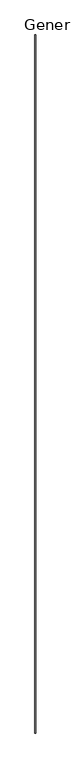
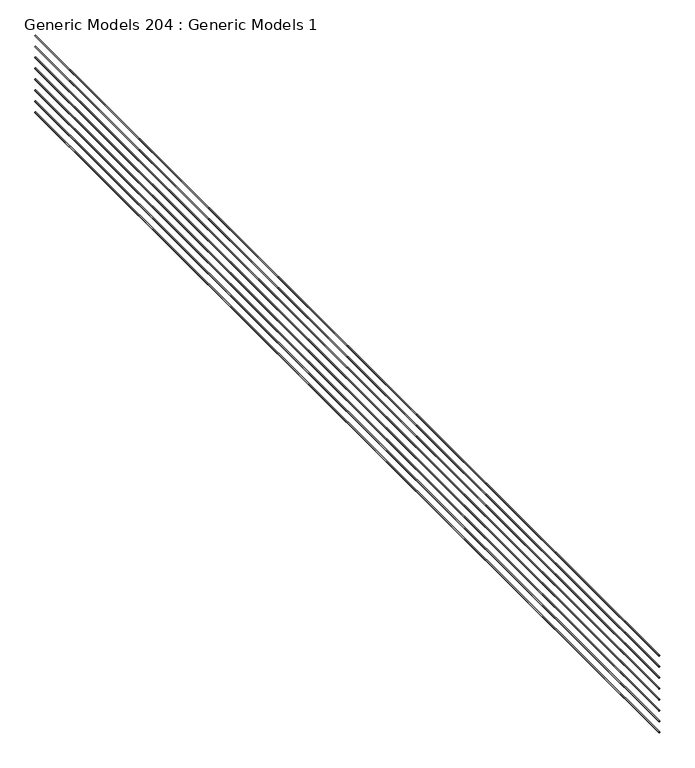
"""IFC4 building model written with IfcOpenShell, lengths in millimetres: proxy geometry, Generic Models 204 : Generic Models 1."""

import ifcopenshell
import ifcopenshell.guid

model = None  # the IFC model being written
_history = None  # IfcOwnerHistory: only IFC2X3 demands one
_inside = {}  # id of a spatial element -> (the spatial element, [elements in it])
_under = {}  # id of a project, library or spatial element -> (it, [spatial elements below it])
_declared = {}  # id of a project -> (the project, [libraries it declares])
_typed = {}  # id of a type object -> (the type object, [elements of that type])
_made_of = {}  # id of a material, layer set ... -> (it, [elements and type objects made of it])


def new_model(schema):
    """Start an empty IFC model of exactly this schema.

    Asked for "IFC4X3", IfcOpenShell would pick the latest addendum, in which some entities
    have other attributes; the version numbers below select the first issue.
    IFC2X3 requires an IfcOwnerHistory on every rooted entity: one is made here for all.
    """
    global model, _history
    if schema == "IFC4X3":
        model = ifcopenshell.file(schema_version=(4, 3, 0, 0))
    else:
        model = ifcopenshell.file(schema=schema)
    _inside.clear()
    _under.clear()
    _declared.clear()
    _typed.clear()
    _made_of.clear()
    _history = None
    if model.schema == "IFC2X3":
        org = make("IfcOrganization", Name="unknown")
        user = make(
            "IfcPersonAndOrganization",
            ThePerson=make("IfcPerson", FamilyName="unknown"),
            TheOrganization=org,
        )
        app = make(
            "IfcApplication",
            ApplicationDeveloper=org,
            Version="unknown",
            ApplicationFullName="unknown",
            ApplicationIdentifier="unknown",
        )
        _history = make(
            "IfcOwnerHistory",
            OwningUser=user,
            OwningApplication=app,
            ChangeAction="ADDED",
            CreationDate=0,
        )
    return model


def make(cls, **values):
    """One entity of the class cls with the attributes given. An attribute that is None is left unset."""
    return model.create_entity(
        cls, **{name: value for name, value in values.items() if value is not None}
    )


def rooted(cls, **values):
    """An entity with a GlobalId (a new one), such as an element, a storey or a relation."""
    return make(cls, GlobalId=ifcopenshell.guid.new(), OwnerHistory=_history, **values)


def si_unit(unit_type, name, prefix=None):
    """IfcSIUnit, for example si_unit("LENGTHUNIT", "METRE", prefix="MILLI")."""
    return make("IfcSIUnit", UnitType=unit_type, Prefix=prefix, Name=name)


def assignment(units):
    """IfcUnitAssignment: the units of a project."""
    return None if units is None else make("IfcUnitAssignment", Units=units)


def point(xyz):
    """IfcCartesianPoint."""
    return None if xyz is None else make("IfcCartesianPoint", Coordinates=xyz)


def direction(xyz):
    """IfcDirection."""
    return None if xyz is None else make("IfcDirection", DirectionRatios=xyz)


def frame(location, z_axis=None, x_axis=None):
    """IfcAxis2Placement3D, a coordinate frame: its origin and axes. An axis left out is left unset."""
    return make(
        "IfcAxis2Placement3D",
        Location=point(location),
        Axis=direction(z_axis),
        RefDirection=direction(x_axis),
    )


def frame_2d(location, x_axis=None):
    """IfcAxis2Placement2D, a coordinate frame in the plane: its origin and x axis."""
    return make(
        "IfcAxis2Placement2D", Location=point(location), RefDirection=direction(x_axis)
    )


def origin():
    """The frame at (0, 0, 0) with its axes left unset."""
    return frame((0.0, 0.0, 0.0))


def place(relative_to, where):
    """IfcLocalPlacement: puts the frame where relative to a parent placement (None: the world)."""
    return make(
        "IfcLocalPlacement", PlacementRelTo=relative_to, RelativePlacement=where
    )


def context(
    kind, dimensions, precision=None, world=None, true_north=None, identifier=None
):
    """IfcGeometricRepresentationContext, for example the 3D "Model" context."""
    return make(
        "IfcGeometricRepresentationContext",
        ContextIdentifier=identifier,
        ContextType=kind,
        CoordinateSpaceDimension=dimensions,
        Precision=precision,
        WorldCoordinateSystem=world,
        TrueNorth=true_north,
    )


def project(units=None, contexts=None):
    """IfcProject with its units and contexts."""
    return rooted(
        "IfcProject",
        Name="project",
        RepresentationContexts=contexts,
        UnitsInContext=assignment(units),
    )


def spatial(cls, under=None, at=None, **own):
    """A site, building, storey or space (cls), placed at a placement, below another one or the project."""
    s = rooted(cls, ObjectPlacement=at, **own)
    if under is not None:
        _under.setdefault(under.id(), (under, []))[1].append(s)
    return s


def circle_curve(where, radius):
    """IfcCircle in the frame where."""
    return make("IfcCircle", Position=where, Radius=radius)


def trimmed(basis, trim1, trim2, sense, master):
    """IfcTrimmedCurve: the piece of a basis curve between two trims."""
    return make(
        "IfcTrimmedCurve",
        BasisCurve=basis,
        Trim1=trim1,
        Trim2=trim2,
        SenseAgreement=sense,
        MasterRepresentation=master,
    )


def segment(curve, same_sense, transition):
    """IfcCompositeCurveSegment."""
    return make(
        "IfcCompositeCurveSegment",
        Transition=transition,
        SameSense=same_sense,
        ParentCurve=curve,
    )


def composite_curve(segments, self_intersect=None):
    """IfcCompositeCurve: segments joined end to end."""
    return make("IfcCompositeCurve", Segments=segments, SelfIntersect=self_intersect)


def outline(outer, holes=None, kind="AREA"):
    """IfcArbitraryClosedProfileDef: a profile drawn as a closed curve; with holes, ...WithVoids."""
    if holes is None:
        return make("IfcArbitraryClosedProfileDef", ProfileType=kind, OuterCurve=outer)
    return make(
        "IfcArbitraryProfileDefWithVoids",
        ProfileType=kind,
        OuterCurve=outer,
        InnerCurves=holes,
    )


def extrude(swept, where, along, depth):
    """IfcExtrudedAreaSolid: the profile swept, set in the frame where, extruded along a direction by depth."""
    return make(
        "IfcExtrudedAreaSolid",
        SweptArea=swept,
        Position=where,
        ExtrudedDirection=direction(along),
        Depth=depth,
    )


def shape(context_of_items, identifier, shape_type, items):
    """IfcShapeRepresentation: the items that make up one representation, for example the "Body"."""
    return make(
        "IfcShapeRepresentation",
        ContextOfItems=context_of_items,
        RepresentationIdentifier=identifier,
        RepresentationType=shape_type,
        Items=items,
    )


def source(mapping_origin, context_of_items, identifier, shape_type, items):
    """IfcRepresentationMap: a shape defined once, which mapped items show again and again."""
    return make(
        "IfcRepresentationMap",
        MappingOrigin=mapping_origin,
        MappedRepresentation=shape(context_of_items, identifier, shape_type, items),
    )


def transform(
    local_origin,
    x_axis=None,
    y_axis=None,
    z_axis=None,
    scale=None,
    scale2=None,
    scale3=None,
    uniform=True,
):
    """IfcCartesianTransformationOperator3D, or its non-uniform kind. x_axis, y_axis, z_axis: its Axis1, 2, 3."""
    if uniform:
        return make(
            "IfcCartesianTransformationOperator3D",
            Axis1=direction(x_axis),
            Axis2=direction(y_axis),
            LocalOrigin=point(local_origin),
            Scale=scale,
            Axis3=direction(z_axis),
        )
    return make(
        "IfcCartesianTransformationOperator3DnonUniform",
        Axis1=direction(x_axis),
        Axis2=direction(y_axis),
        LocalOrigin=point(local_origin),
        Scale=scale,
        Axis3=direction(z_axis),
        Scale2=scale2,
        Scale3=scale3,
    )


def mapped(mapping_source, mapping_target):
    """IfcMappedItem: shows the shape of a source again, moved by a transform."""
    return make(
        "IfcMappedItem", MappingSource=mapping_source, MappingTarget=mapping_target
    )


def made_of(thing, what):
    """Note that an element or type object is made of a material, layer set ...; save() writes the relation."""
    if what is not None:
        _made_of.setdefault(what.id(), (what, []))[1].append(thing)
    return thing


def element(
    cls,
    number,
    at=None,
    inside=None,
    cuts=None,
    type_object=None,
    material=None,
    context=None,
    identifier="Body",
    shape_type=None,
    held_by="IfcProductDefinitionShape",
    body=None,
    shapes=None,
    **own,
):
    """One element of the class cls, such as IfcWall. Its Tag is "e" and its number.

    at: its placement. inside: the storey or other place that contains it. cuts: it is an
    opening in that element (IfcRelVoidsElement). A single representation is given by context,
    identifier, shape_type and body (its items); several are given by shapes. held_by: the class
    of the entity that holds the representations. save() writes the other relations.
    """
    e = rooted(cls, Tag="e%d" % number, ObjectPlacement=at, **own)
    if body is not None:
        shapes = [shape(context, identifier, shape_type, body)]
    if shapes is not None:
        e.Representation = make(held_by, Representations=shapes)
    if inside is not None:
        _inside.setdefault(inside.id(), (inside, []))[1].append(e)
    if cuts is not None:
        rooted(
            "IfcRelVoidsElement", RelatingBuildingElement=cuts, RelatedOpeningElement=e
        )
    if type_object is not None:
        _typed.setdefault(type_object.id(), (type_object, []))[1].append(e)
    return made_of(e, material)


def aggregate(whole, parts):
    """IfcRelAggregates: a whole, such as a stair, and the parts it consists of."""
    return rooted("IfcRelAggregates", RelatingObject=whole, RelatedObjects=parts)


def save(model, path):
    """Write the relations noted so far, then the file.

    IfcRelAggregates (storeys below a building ...), IfcRelContainedInSpatialStructure (elements
    in a storey), IfcRelDefinesByType, IfcRelAssociatesMaterial and IfcRelDeclares: one each for
    every whole, place, type object, material and project.
    """
    for whole, parts in _under.values():
        aggregate(whole, parts)
    for where, things in _inside.values():
        rooted(
            "IfcRelContainedInSpatialStructure",
            RelatedElements=things,
            RelatingStructure=where,
        )
    for kind, things in _typed.values():
        rooted("IfcRelDefinesByType", RelatedObjects=things, RelatingType=kind)
    for what, things in _made_of.values():
        rooted("IfcRelAssociatesMaterial", RelatedObjects=things, RelatingMaterial=what)
    for by, libraries in _declared.values():
        rooted("IfcRelDeclares", RelatingContext=by, RelatedDefinitions=libraries)
    model.write(path)


def generic_models_204_generic_models_1_ff4490ce(model_context):
    return source(origin(), model_context, "Body", "SweptSolid", [
        extrude(outline(composite_curve([segment(trimmed(circle_curve(frame_2d((127752.221, -8255.1736296)), 4.7625), [point((127752.221, -8259.9361296))], [point((127752.221, -8250.4111296))], False, "CARTESIAN"), True, "CONTINUOUS"), segment(trimmed(circle_curve(frame_2d((127752.221, -8255.1736296)), 4.7625), [point((127752.221, -8250.4111296))], [point((127752.221, -8259.9361296))], False, "CARTESIAN"), True, "CONTINUOUS")], self_intersect=False)), frame((0.0, -654.6230338, 0.0), z_axis=(0.0, 1.0, 0.0), x_axis=(0.0, 0.0, 1.0)), (0.0, 0.0, 1.0), 9475.7774227),
        extrude(outline(composite_curve([segment(trimmed(circle_curve(frame_2d((127650.621, -8255.1736296)), 4.7625), [point((127650.621, -8259.9361296))], [point((127650.621, -8250.4111296))], False, "CARTESIAN"), True, "CONTINUOUS"), segment(trimmed(circle_curve(frame_2d((127650.621, -8255.1736296)), 4.7625), [point((127650.621, -8250.4111296))], [point((127650.621, -8259.9361296))], False, "CARTESIAN"), True, "CONTINUOUS")], self_intersect=False)), frame((0.0, -654.6230338, 0.0), z_axis=(0.0, 1.0, 0.0), x_axis=(0.0, 0.0, 1.0)), (0.0, 0.0, 1.0), 9475.7774227),
        extrude(outline(composite_curve([segment(trimmed(circle_curve(frame_2d((127549.021, -8255.1736296)), 4.7625), [point((127549.021, -8259.9361296))], [point((127549.021, -8250.4111296))], False, "CARTESIAN"), True, "CONTINUOUS"), segment(trimmed(circle_curve(frame_2d((127549.021, -8255.1736296)), 4.7625), [point((127549.021, -8250.4111296))], [point((127549.021, -8259.9361296))], False, "CARTESIAN"), True, "CONTINUOUS")], self_intersect=False)), frame((0.0, -654.6230338, 0.0), z_axis=(0.0, 1.0, 0.0), x_axis=(0.0, 0.0, 1.0)), (0.0, 0.0, 1.0), 9475.7774227),
        extrude(outline(composite_curve([segment(trimmed(circle_curve(frame_2d((127447.421, -8255.1736296)), 4.7625), [point((127447.421, -8259.9361296))], [point((127447.421, -8250.4111296))], False, "CARTESIAN"), True, "CONTINUOUS"), segment(trimmed(circle_curve(frame_2d((127447.421, -8255.1736296)), 4.7625), [point((127447.421, -8250.4111296))], [point((127447.421, -8259.9361296))], False, "CARTESIAN"), True, "CONTINUOUS")], self_intersect=False)), frame((0.0, -654.6230338, 0.0), z_axis=(0.0, 1.0, 0.0), x_axis=(0.0, 0.0, 1.0)), (0.0, 0.0, 1.0), 9475.7774227),
        extrude(outline(composite_curve([segment(trimmed(circle_curve(frame_2d((127345.821, -8255.1736296)), 4.7625), [point((127345.821, -8259.9361296))], [point((127345.821, -8250.4111296))], False, "CARTESIAN"), True, "CONTINUOUS"), segment(trimmed(circle_curve(frame_2d((127345.821, -8255.1736296)), 4.7625), [point((127345.821, -8250.4111296))], [point((127345.821, -8259.9361296))], False, "CARTESIAN"), True, "CONTINUOUS")], self_intersect=False)), frame((0.0, -654.6230338, 0.0), z_axis=(0.0, 1.0, 0.0), x_axis=(0.0, 0.0, 1.0)), (0.0, 0.0, 1.0), 9475.7774227),
        extrude(outline(composite_curve([segment(trimmed(circle_curve(frame_2d((127244.221, -8255.1736296)), 4.7625), [point((127244.221, -8259.9361296))], [point((127244.221, -8250.4111296))], False, "CARTESIAN"), True, "CONTINUOUS"), segment(trimmed(circle_curve(frame_2d((127244.221, -8255.1736296)), 4.7625), [point((127244.221, -8250.4111296))], [point((127244.221, -8259.9361296))], False, "CARTESIAN"), True, "CONTINUOUS")], self_intersect=False)), frame((0.0, -654.6230338, 0.0), z_axis=(0.0, 1.0, 0.0), x_axis=(0.0, 0.0, 1.0)), (0.0, 0.0, 1.0), 9475.7774227),
        extrude(outline(composite_curve([segment(trimmed(circle_curve(frame_2d((127142.621, -8255.1736296)), 4.7625), [point((127142.621, -8259.9361296))], [point((127142.621, -8250.4111296))], False, "CARTESIAN"), True, "CONTINUOUS"), segment(trimmed(circle_curve(frame_2d((127142.621, -8255.1736296)), 4.7625), [point((127142.621, -8250.4111296))], [point((127142.621, -8259.9361296))], False, "CARTESIAN"), True, "CONTINUOUS")], self_intersect=False)), frame((0.0, -654.6230338, 0.0), z_axis=(0.0, 1.0, 0.0), x_axis=(0.0, 0.0, 1.0)), (0.0, 0.0, 1.0), 9475.7774227),
        extrude(outline(composite_curve([segment(trimmed(circle_curve(frame_2d((127041.021, -8255.1736296)), 4.7625), [point((127041.021, -8259.9361296))], [point((127041.021, -8250.4111296))], False, "CARTESIAN"), True, "CONTINUOUS"), segment(trimmed(circle_curve(frame_2d((127041.021, -8255.1736296)), 4.7625), [point((127041.021, -8250.4111296))], [point((127041.021, -8259.9361296))], False, "CARTESIAN"), True, "CONTINUOUS")], self_intersect=False)), frame((0.0, -654.6230338, 0.0), z_axis=(0.0, 1.0, 0.0), x_axis=(0.0, 0.0, 1.0)), (0.0, 0.0, 1.0), 9475.7774227),
    ])


if __name__ == "__main__":
    model = new_model("IFC4")
    model_context = context("Model", 3, world=origin())
    ifc_project = project(units=[si_unit("LENGTHUNIT", "METRE", prefix="MILLI")], contexts=[model_context])
    site = spatial("IfcSite", under=ifc_project)
    building = spatial("IfcBuilding", under=site)
    placement = place(None, origin())
    generic_models_204_generic_models_1_shape = generic_models_204_generic_models_1_ff4490ce(model_context)
    element("IfcBuildingElementProxy", 1, Name="Generic Models 204 : Generic Models 1", ObjectType="Generic Models 204 : Generic Models 1", at=placement, inside=building, context=model_context, shape_type="MappedRepresentation", body=[
        mapped(generic_models_204_generic_models_1_shape, transform((0.0, 0.0, 0.0), x_axis=(1.0, 0.0, 0.0), y_axis=(0.0, 1.0, 0.0), z_axis=(0.0, 0.0, 1.0))),
    ])
    save(model, "model.ifc")

# Revit data of these elements
# Element 1 (IfcBuildingElementProxy, "Generic Models 204 : Generic Models 1")
#   Materials on its faces: "_1/2\" DIA. SOLID STOCK STEEL HORIZONTAL RAILINGS"
# Materials
#   "_1/2\" DIA. SOLID STOCK STEEL HORIZONTAL RAILINGS": class "Metal", colour RGB 199 199 199, transparency 0, Description = "Structural steel 50ksi", Cost = 0
